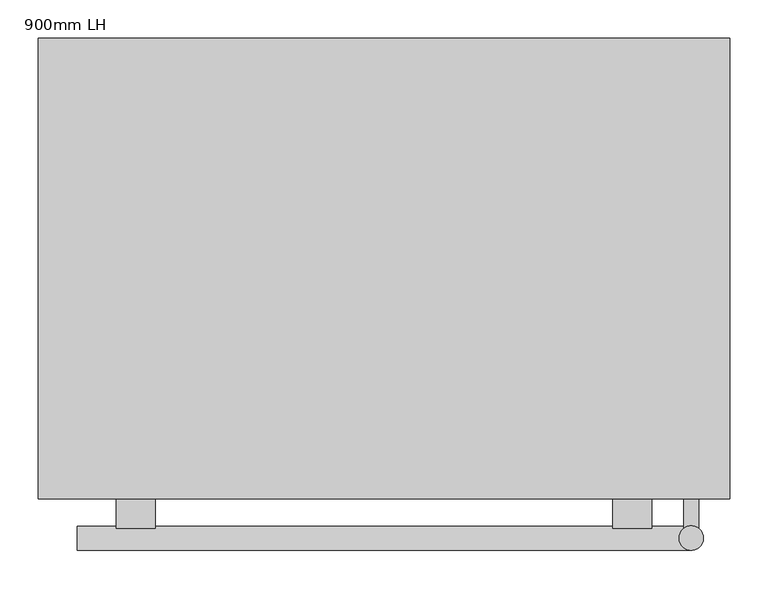
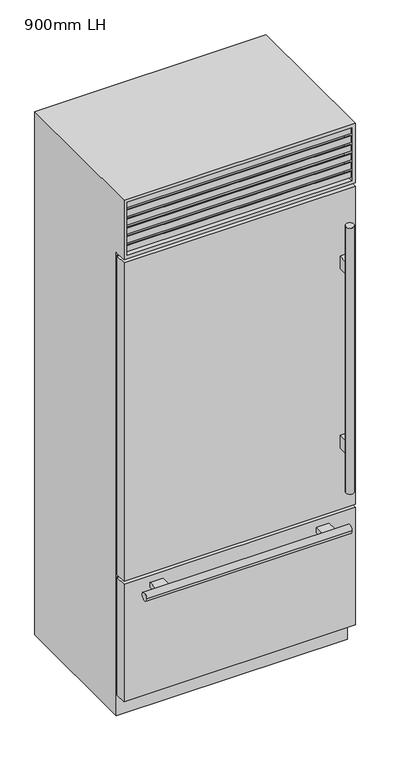
"""IFC4 building model written with IfcOpenShell, lengths in millimetres: proxy geometry, Refrigerador-combinado : 900mm LH."""

from ifc_helpers import new_model, si_unit, frame, origin, place, context, project, spatial, polyline, circle_curve, ellipse_curve, outline, extrude, faceted_brep, source, transform, mapped, element, save
from ifc_brep_helpers import plane_surface, cylinder_surface, advanced_brep


def proxy_900mm_lh_87200827(model_context):
    return source(origin(), model_context, "Body", "SolidModel", [
        extrude(outline(polyline([(-450.0, -655.55), (450.0, -655.55), (450.0, -700.0), (-450.0, -700.0), (-450.0, -655.55)])), frame((0.0, 0.0, 584.2), z_axis=(0.0, 0.0, 1.0), x_axis=(1.0, 0.0, 0.0)), (0.0, 0.0, 1.0), 1308.625),
        extrude(outline(polyline([(-450.0, -655.55), (450.0, -655.55), (450.0, -700.0), (-450.0, -700.0), (-450.0, -655.55)])), frame((0.0, 0.0, 88.9), z_axis=(0.0, 0.0, 1.0), x_axis=(1.0, 0.0, 0.0)), (0.0, 0.0, 1.0), 482.6),
        faceted_brep([(450.0, -700.0, 2150.0), (-450.0, -700.0, 2150.0), (-450.0, -700.0, 1905.525), (450.0, -700.0, 1905.525), (437.3, -700.0, 2137.3), (437.3, -700.0, 1918.225), (-437.3, -700.0, 1918.225), (-437.3, -700.0, 2137.3), (450.0, -100.0, 2150.0), (-450.0, -100.0, 2150.0), (-450.0, -100.0, 0.0), (-450.0, -649.2, 0.0), (-450.0, -649.2, 1905.525), (450.0, -649.2, 1905.525), (450.0, -649.2, 0.0), (450.0, -100.0, 0.0), (-437.3, -649.2, 2137.3), (437.3, -649.2, 2137.3), (-437.3, -649.2, 1918.225), (437.3, -649.2, 1918.225)], [[[0, 1, 2, 3], [4, 5, 6, 7]], [[1, 0, 8, 9]], [[2, 1, 9, 10, 11, 12]], [[3, 2, 12, 13]], [[8, 0, 3, 13, 14, 15]], [[4, 7, 16, 17]], [[7, 6, 18, 16]], [[6, 5, 19, 18]], [[5, 4, 17, 19]], [[15, 14, 11, 10]], [[9, 8, 15, 10]], [[17, 16, 18, 19]], [[11, 14, 13, 12]]]),
        extrude(outline(polyline([(-649.2, 1918.225), (-696.825, 1930.9860803), (-696.825, 1956.3860803), (-693.65, 1956.3860803), (-693.65, 1933.5368938), (-649.2, 1921.6265522), (-649.2, 1918.225)])), frame((-437.3, 0.0, 0.0), z_axis=(1.0, 0.0, 0.0), x_axis=(0.0, 1.0, 0.0)), (0.0, 0.0, 1.0), 874.6),
        extrude(outline(polyline([(-649.2, 1954.4077839), (-696.825, 1967.1688642), (-696.825, 1992.5688642), (-693.65, 1992.5688642), (-693.65, 1969.7196777), (-649.2, 1957.8093361), (-649.2, 1954.4077839)])), frame((-437.3, 0.0, 0.0), z_axis=(1.0, 0.0, 0.0), x_axis=(0.0, 1.0, 0.0)), (0.0, 0.0, 1.0), 874.6),
        extrude(outline(polyline([(-649.2, 1990.5905679), (-696.825, 2003.3516482), (-696.825, 2028.7516482), (-693.65, 2028.7516482), (-693.65, 2005.9024616), (-649.2, 1993.99212), (-649.2, 1990.5905679)])), frame((-437.3, 0.0, 0.0), z_axis=(1.0, 0.0, 0.0), x_axis=(0.0, 1.0, 0.0)), (0.0, 0.0, 1.0), 874.6),
        extrude(outline(polyline([(-649.2, 2026.7733518), (-696.825, 2039.5344321), (-696.825, 2064.9344321), (-693.65, 2064.9344321), (-693.65, 2042.0852456), (-649.2, 2030.174904), (-649.2, 2026.7733518)])), frame((-437.3, 0.0, 0.0), z_axis=(1.0, 0.0, 0.0), x_axis=(0.0, 1.0, 0.0)), (0.0, 0.0, 1.0), 874.6),
        extrude(outline(polyline([(-649.2, 2062.9561358), (-696.825, 2075.7172161), (-696.825, 2101.1172161), (-693.65, 2101.1172161), (-693.65, 2078.2680295), (-649.2, 2066.3576879), (-649.2, 2062.9561358)])), frame((-437.3, 0.0, 0.0), z_axis=(1.0, 0.0, 0.0), x_axis=(0.0, 1.0, 0.0)), (0.0, 0.0, 1.0), 874.6),
        extrude(outline(polyline([(-649.2, 2099.1389197), (-696.825, 2111.9), (-696.825, 2137.3), (-693.65, 2137.3), (-693.65, 2114.4508135), (-649.2, 2102.5404719), (-649.2, 2099.1389197)])), frame((-437.3, 0.0, 0.0), z_axis=(1.0, 0.0, 0.0), x_axis=(0.0, 1.0, 0.0)), (0.0, 0.0, 1.0), 874.6),
        advanced_brep(
        [(-443.65, -649.2, 565.15), (-443.65, -655.55, 565.15), (-443.65, -655.55, 95.25), (-443.65, -649.2, 95.25), (-446.825, -655.55, 568.325), (-446.825, -649.2, 568.325), (-446.825, -649.2, 92.075), (-446.825, -655.55, 92.075), (443.65, -655.55, 95.25), (443.65, -649.2, 95.25), (446.825, -649.2, 92.075), (446.825, -655.55, 92.075), (443.65, -655.55, 565.15), (443.65, -649.2, 565.15), (446.825, -649.2, 568.325), (446.825, -655.55, 568.325)],
        [
            (0, 1),
            (1, 2),
            (2, 3),
            (3, 0),
            (4, 5, ellipse_curve(frame((-446.825, -652.375, 568.325), z_axis=(-0.7071067811865475, 0.0, -0.7071067811865476), x_axis=(-0.7071067811865476, 0.0, 0.7071067811865475)), 4.4901281, 3.175)),
            (5, 6),
            (6, 7, ellipse_curve(frame((-446.825, -652.375, 92.075), z_axis=(-0.7071067811865475, 0.0, 0.7071067811865475), x_axis=(0.7071067811865474, 0.0, 0.7071067811865477)), 4.4901281, 3.175)),
            (7, 4),
            (2, 8),
            (8, 9),
            (9, 3),
            (6, 10),
            (10, 11, ellipse_curve(frame((446.825, -652.375, 92.075), z_axis=(-0.7071067811865475, 0.0, -0.7071067811865476), x_axis=(-0.7071067811865476, 0.0, 0.7071067811865474)), 4.4901281, 3.175)),
            (11, 7),
            (8, 12),
            (12, 13),
            (13, 9),
            (10, 14),
            (14, 15, ellipse_curve(frame((446.825, -652.375, 568.325), z_axis=(0.7071067811865476, 0.0, -0.7071067811865474), x_axis=(-0.7071067811865474, 0.0, -0.7071067811865477)), 4.4901281, 3.175)),
            (15, 11),
            (12, 1),
            (0, 13),
            (5, 14),
            (4, 15),
        ],
        [
            plane_surface(frame((-443.65, -655.55, 565.15), z_axis=(1.0, 0.0, 0.0), x_axis=(0.0, 0.0, -1.0))),
            cylinder_surface(frame((-446.825, -652.375, 571.5), z_axis=(0.0, 0.0, 1.0), x_axis=(0.0, -1.0, 0.0)), 3.175),
            plane_surface(frame((-443.65, -655.55, 95.25), z_axis=(0.0, 0.0, 1.0), x_axis=(1.0, 0.0, 0.0))),
            cylinder_surface(frame((-450.0, -652.375, 92.075), z_axis=(-1.0, 0.0, 0.0), x_axis=(0.0, -1.0, 0.0)), 3.175),
            plane_surface(frame((443.65, -655.55, 95.25), z_axis=(-1.0, 0.0, 0.0), x_axis=(0.0, 0.0, 1.0))),
            cylinder_surface(frame((446.825, -652.375, 88.9), z_axis=(0.0, 0.0, -1.0), x_axis=(0.0, -1.0, 0.0)), 3.175),
            plane_surface(frame((443.65, -655.55, 565.15), z_axis=(0.0, 0.0, -1.0), x_axis=(-1.0, 0.0, 0.0))),
            plane_surface(frame((443.65, -649.2, 565.15), z_axis=(0.0, 1.0, 0.0), x_axis=(-1.0, 0.0, 0.0))),
            cylinder_surface(frame((450.0, -652.375, 568.325), z_axis=(1.0, 0.0, 0.0), x_axis=(0.0, -1.0, 0.0)), 3.175),
            plane_surface(frame((446.825, -655.55, 568.325), z_axis=(0.0, -1.0, 0.0), x_axis=(-1.0, 0.0, 0.0))),
        ],
        [
            (0, [[1, 2, 3, 4]]),
            (1, [[5, 6, 7, 8]]),
            (2, [[-3, 9, 10, 11]]),
            (3, [[-7, 12, 13, 14]]),
            (4, [[-10, 15, 16, 17]]),
            (5, [[-13, 18, 19, 20]]),
            (6, [[-16, 21, -1, 22]]),
            (7, [[23, -18, -12, -6], [-11, -17, -22, -4]]),
            (8, [[-19, -23, -5, 24]]),
            (9, [[-14, -20, -24, -8], [-21, -15, -9, -2]]),
        ],
    ),
        advanced_brep(
        [(-443.65, -649.2, 1886.475), (-443.65, -655.55, 1886.475), (-443.65, -655.55, 590.55), (-443.65, -649.2, 590.55), (-446.825, -655.55, 1889.65), (-446.825, -649.2, 1889.65), (-446.825, -649.2, 587.375), (-446.825, -655.55, 587.375), (443.65, -655.55, 590.55), (443.65, -649.2, 590.55), (446.825, -649.2, 587.375), (446.825, -655.55, 587.375), (443.65, -655.55, 1886.475), (443.65, -649.2, 1886.475), (446.825, -649.2, 1889.65), (446.825, -655.55, 1889.65)],
        [
            (0, 1),
            (1, 2),
            (2, 3),
            (3, 0),
            (4, 5, ellipse_curve(frame((-446.825, -652.375, 1889.65), z_axis=(-0.7071067811865476, 0.0, -0.7071067811865475), x_axis=(-0.7071067811865475, 0.0, 0.7071067811865475)), 4.4901281, 3.175)),
            (5, 6),
            (6, 7, ellipse_curve(frame((-446.825, -652.375, 587.375), z_axis=(-0.7071067811865475, 0.0, 0.7071067811865476), x_axis=(0.7071067811865475, 0.0, 0.7071067811865475)), 4.4901281, 3.175)),
            (7, 4),
            (2, 8),
            (8, 9),
            (9, 3),
            (6, 10),
            (10, 11, ellipse_curve(frame((446.825, -652.375, 587.375), z_axis=(-0.7071067811865476, 0.0, -0.7071067811865475), x_axis=(-0.7071067811865475, 0.0, 0.7071067811865475)), 4.4901281, 3.175)),
            (11, 7),
            (8, 12),
            (12, 13),
            (13, 9),
            (10, 14),
            (14, 15, ellipse_curve(frame((446.825, -652.375, 1889.65), z_axis=(0.7071067811865474, 0.0, -0.7071067811865476), x_axis=(-0.7071067811865475, 0.0, -0.7071067811865476)), 4.4901281, 3.175)),
            (15, 11),
            (12, 1),
            (0, 13),
            (5, 14),
            (4, 15),
        ],
        [
            plane_surface(frame((-443.65, -655.55, 1886.475), z_axis=(1.0, 0.0, 0.0), x_axis=(0.0, 0.0, -1.0))),
            cylinder_surface(frame((-446.825, -652.375, 1892.825), z_axis=(0.0, 0.0, 1.0), x_axis=(0.0, -1.0, 0.0)), 3.175),
            plane_surface(frame((-443.65, -655.55, 590.55), z_axis=(0.0, 0.0, 1.0), x_axis=(1.0, 0.0, 0.0))),
            cylinder_surface(frame((-450.0, -652.375, 587.375), z_axis=(-1.0, 0.0, 0.0), x_axis=(0.0, -1.0, 0.0)), 3.175),
            plane_surface(frame((443.65, -655.55, 590.55), z_axis=(-1.0, 0.0, 0.0), x_axis=(0.0, 0.0, 1.0))),
            cylinder_surface(frame((446.825, -652.375, 584.2), z_axis=(0.0, 0.0, -1.0), x_axis=(0.0, -1.0, 0.0)), 3.175),
            plane_surface(frame((443.65, -655.55, 1886.475), z_axis=(0.0, 0.0, -1.0), x_axis=(-1.0, 0.0, 0.0))),
            plane_surface(frame((443.65, -649.2, 1886.475), z_axis=(0.0, 1.0, 0.0), x_axis=(-1.0, 0.0, 0.0))),
            cylinder_surface(frame((450.0, -652.375, 1889.65), z_axis=(1.0, 0.0, 0.0), x_axis=(0.0, -1.0, 0.0)), 3.175),
            plane_surface(frame((446.825, -655.55, 1889.65), z_axis=(0.0, -1.0, 0.0), x_axis=(-1.0, 0.0, 0.0))),
        ],
        [
            (0, [[1, 2, 3, 4]]),
            (1, [[5, 6, 7, 8]]),
            (2, [[-3, 9, 10, 11]]),
            (3, [[-7, 12, 13, 14]]),
            (4, [[-10, 15, 16, 17]]),
            (5, [[-13, 18, 19, 20]]),
            (6, [[-16, 21, -1, 22]]),
            (7, [[23, -18, -12, -6], [-11, -17, -22, -4]]),
            (8, [[-19, -23, -5, 24]]),
            (9, [[-14, -20, -24, -8], [-21, -15, -9, -2]]),
        ],
    ),
        advanced_brep(
        [(-297.6, -700.0, 542.925), (-297.6, -700.0, 523.875), (-348.4, -700.0, 523.875), (-348.4, -700.0, 542.925), (297.6, -700.0, 542.925), (348.4, -700.0, 542.925), (348.4, -700.0, 523.875), (297.6, -700.0, 523.875), (-297.6, -738.4741958, 542.925), (-297.6, -735.2991958, 533.4), (-297.6, -738.4741958, 523.875), (-348.4, -738.4741958, 523.875), (-348.4, -735.2991958, 533.4), (-348.4, -738.4741958, 542.925), (297.6, -738.4741958, 542.925), (348.4, -738.4741958, 542.925), (348.4, -735.2991958, 533.4), (348.4, -738.4741958, 523.875), (297.6, -738.4741958, 523.875), (297.6, -735.2991958, 533.4), (399.2, -767.0491958, 533.4), (399.2, -735.2991958, 533.4), (-399.2, -767.0491958, 533.4), (-399.2, -735.2991958, 533.4)],
        [
            (0, 1),
            (1, 2),
            (2, 3),
            (3, 0),
            (4, 5),
            (5, 6),
            (6, 7),
            (7, 4),
            (0, 8),
            (8, 9, circle_curve(frame((-297.6, -751.1741958, 533.4), z_axis=(-1.0, 0.0, 0.0), x_axis=(0.0, 1.0, 0.0)), 15.875)),
            (9, 10, circle_curve(frame((-297.6, -751.1741958, 533.4), z_axis=(-1.0, 0.0, 0.0), x_axis=(0.0, 1.0, 0.0)), 15.875)),
            (10, 1),
            (10, 11),
            (11, 2),
            (11, 12, circle_curve(frame((-348.4, -751.1741958, 533.4), z_axis=(1.0, 0.0, 0.0), x_axis=(0.0, 1.0, 0.0)), 15.875)),
            (12, 13, circle_curve(frame((-348.4, -751.1741958, 533.4), z_axis=(1.0, 0.0, 0.0), x_axis=(0.0, 1.0, 0.0)), 15.875)),
            (13, 3),
            (13, 8),
            (4, 14),
            (14, 15),
            (15, 5),
            (15, 16, circle_curve(frame((348.4, -751.1741958, 533.4), z_axis=(-1.0, 0.0, 0.0), x_axis=(0.0, 1.0, 0.0)), 15.875)),
            (16, 17, circle_curve(frame((348.4, -751.1741958, 533.4), z_axis=(-1.0, 0.0, 0.0), x_axis=(0.0, 1.0, 0.0)), 15.875)),
            (17, 6),
            (17, 18),
            (18, 7),
            (18, 19, circle_curve(frame((297.6, -751.1741958, 533.4), z_axis=(1.0, 0.0, 0.0), x_axis=(0.0, 1.0, 0.0)), 15.875)),
            (19, 14, circle_curve(frame((297.6, -751.1741958, 533.4), z_axis=(1.0, 0.0, 0.0), x_axis=(0.0, 1.0, 0.0)), 15.875)),
            (20, 21, circle_curve(frame((399.2, -751.1741958, 533.4), z_axis=(1.0, 0.0, 0.0), x_axis=(0.0, 1.0, 0.0)), 15.875)),
            (21, 20, circle_curve(frame((399.2, -751.1741958, 533.4), z_axis=(1.0, 0.0, 0.0), x_axis=(0.0, 1.0, 0.0)), 15.875)),
            (22, 23, circle_curve(frame((-399.2, -751.1741958, 533.4), z_axis=(-1.0, 0.0, 0.0), x_axis=(0.0, 1.0, 0.0)), 15.875)),
            (23, 22, circle_curve(frame((-399.2, -751.1741958, 533.4), z_axis=(-1.0, 0.0, 0.0), x_axis=(0.0, 1.0, 0.0)), 15.875)),
            (20, 22),
            (23, 12),
            (9, 19),
            (16, 21),
        ],
        [
            plane_surface(frame((-297.6, -700.0, 542.925), z_axis=(0.0, 1.0, 0.0), x_axis=(0.0, 0.0, -1.0))),
            plane_surface(frame((-297.6, -700.0, 542.925), z_axis=(1.0, 0.0, 0.0), x_axis=(0.0, -1.0, 0.0))),
            plane_surface(frame((-297.6, -700.0, 523.875), z_axis=(0.0, 0.0, -1.0), x_axis=(0.0, -1.0, 0.0))),
            plane_surface(frame((-348.4, -700.0, 523.875), z_axis=(-1.0, 0.0, 0.0), x_axis=(0.0, -1.0, 0.0))),
            plane_surface(frame((-348.4, -700.0, 542.925), z_axis=(0.0, 0.0, 1.0), x_axis=(0.0, -1.0, 0.0))),
            plane_surface(frame((297.6, -700.0, 542.925), z_axis=(0.0, 0.0, 1.0), x_axis=(0.0, -1.0, 0.0))),
            plane_surface(frame((348.4, -700.0, 542.925), z_axis=(1.0, 0.0, 0.0), x_axis=(0.0, -1.0, 0.0))),
            plane_surface(frame((348.4, -700.0, 523.875), z_axis=(0.0, 0.0, -1.0), x_axis=(0.0, -1.0, 0.0))),
            plane_surface(frame((297.6, -700.0, 523.875), z_axis=(-1.0, 0.0, 0.0), x_axis=(0.0, -1.0, 0.0))),
            plane_surface(frame((399.2, -735.2991958, 533.4), z_axis=(1.0, 0.0, 0.0), x_axis=(0.0, 0.0, 1.0))),
            plane_surface(frame((-399.2, -735.2991958, 533.4), z_axis=(-1.0, 0.0, 0.0), x_axis=(0.0, 0.0, -1.0))),
            cylinder_surface(frame((-399.2, -751.1741958, 533.4), z_axis=(1.0, 0.0, 0.0), x_axis=(0.0, 1.0, 0.0)), 15.875),
        ],
        [
            (0, [[1, 2, 3, 4]]),
            (0, [[5, 6, 7, 8]]),
            (1, [[-1, 9, 10, 11, 12]]),
            (2, [[-2, -12, 13, 14]]),
            (3, [[-3, -14, 15, 16, 17]]),
            (4, [[-4, -17, 18, -9]]),
            (5, [[-5, 19, 20, 21]]),
            (6, [[-6, -21, 22, 23, 24]]),
            (7, [[-7, -24, 25, 26]]),
            (8, [[-8, -26, 27, 28, -19]]),
            (9, [[29, 30]]),
            (10, [[31, 32]]),
            (11, [[-29, 33, -32, 34, -15, -13, -11, 35, -27, -25, -23, 36]]),
            (11, [[-30, -36, -22, -20, -28, -35, -10, -18, -16, -34, -31, -33]]),
        ],
    ),
        advanced_brep(
        [(409.525, -700.0, 1626.125), (409.525, -700.0, 1575.325), (390.475, -700.0, 1575.325), (390.475, -700.0, 1626.125), (409.525, -700.0, 889.0), (409.525, -700.0, 838.2), (390.475, -700.0, 838.2), (390.475, -700.0, 889.0), (409.525, -738.4741958, 1626.125), (409.525, -738.4741958, 1575.325), (390.475, -738.4741958, 1575.325), (390.475, -738.4741958, 1626.125), (409.525, -738.4741958, 889.0), (409.525, -738.4741958, 838.2), (390.475, -738.4741958, 838.2), (390.475, -738.4741958, 889.0), (384.125, -751.1741958, 1778.525), (415.875, -751.1741958, 1778.525), (384.125, -751.1741958, 685.8), (415.875, -751.1741958, 685.8)],
        [
            (0, 1),
            (1, 2),
            (2, 3),
            (3, 0),
            (4, 5),
            (5, 6),
            (6, 7),
            (7, 4),
            (0, 8),
            (8, 9),
            (9, 1),
            (9, 10, circle_curve(frame((400.0, -751.1741958, 1575.325), z_axis=(0.0, 0.0, 1.0), x_axis=(1.0, 0.0, 0.0)), 15.875)),
            (10, 2),
            (10, 11),
            (11, 3),
            (11, 8, circle_curve(frame((400.0, -751.1741958, 1626.125), z_axis=(0.0, 0.0, -1.0), x_axis=(1.0, 0.0, 0.0)), 15.875)),
            (4, 12),
            (12, 13),
            (13, 5),
            (13, 14, circle_curve(frame((400.0, -751.1741958, 838.2), z_axis=(0.0, 0.0, 1.0), x_axis=(1.0, 0.0, 0.0)), 15.875)),
            (14, 6),
            (14, 15),
            (15, 7),
            (15, 12, circle_curve(frame((400.0, -751.1741958, 889.0), z_axis=(0.0, 0.0, -1.0), x_axis=(1.0, 0.0, 0.0)), 15.875)),
            (16, 17, circle_curve(frame((400.0, -751.1741958, 1778.525), z_axis=(0.0, 0.0, 1.0), x_axis=(1.0, 0.0, 0.0)), 15.875)),
            (17, 16, circle_curve(frame((400.0, -751.1741958, 1778.525), z_axis=(0.0, 0.0, 1.0), x_axis=(1.0, 0.0, 0.0)), 15.875)),
            (18, 19, circle_curve(frame((400.0, -751.1741958, 685.8), z_axis=(0.0, 0.0, -1.0), x_axis=(1.0, 0.0, 0.0)), 15.875)),
            (19, 18, circle_curve(frame((400.0, -751.1741958, 685.8), z_axis=(0.0, 0.0, -1.0), x_axis=(1.0, 0.0, 0.0)), 15.875)),
            (16, 18),
            (19, 17),
        ],
        [
            plane_surface(frame((409.525, -700.0, 1626.125), z_axis=(0.0, 1.0, 0.0), x_axis=(0.0, 0.0, -1.0))),
            plane_surface(frame((409.525, -700.0, 1626.125), z_axis=(1.0, 0.0, 0.0), x_axis=(0.0, -1.0, 0.0))),
            plane_surface(frame((409.525, -700.0, 1575.325), z_axis=(0.0, 0.0, -1.0), x_axis=(0.0, -1.0, 0.0))),
            plane_surface(frame((390.475, -700.0, 1575.325), z_axis=(-1.0, 0.0, 0.0), x_axis=(0.0, -1.0, 0.0))),
            plane_surface(frame((390.475, -700.0, 1626.125), z_axis=(0.0, 0.0, 1.0), x_axis=(0.0, -1.0, 0.0))),
            plane_surface(frame((409.525, -700.0, 889.0), z_axis=(1.0, 0.0, 0.0), x_axis=(0.0, -1.0, 0.0))),
            plane_surface(frame((409.525, -700.0, 838.2), z_axis=(0.0, 0.0, -1.0), x_axis=(0.0, -1.0, 0.0))),
            plane_surface(frame((390.475, -700.0, 838.2), z_axis=(-1.0, 0.0, 0.0), x_axis=(0.0, -1.0, 0.0))),
            plane_surface(frame((390.475, -700.0, 889.0), z_axis=(0.0, 0.0, 1.0), x_axis=(0.0, -1.0, 0.0))),
            plane_surface(frame((415.875, -751.1741958, 1778.525), z_axis=(0.0, 0.0, 1.0), x_axis=(0.0, 1.0, 0.0))),
            plane_surface(frame((415.875, -751.1741958, 685.8), z_axis=(0.0, 0.0, -1.0), x_axis=(0.0, -1.0, 0.0))),
            cylinder_surface(frame((400.0, -751.1741958, 685.8), z_axis=(0.0, 0.0, 1.0), x_axis=(1.0, 0.0, 0.0)), 15.875),
        ],
        [
            (0, [[1, 2, 3, 4]]),
            (0, [[5, 6, 7, 8]]),
            (1, [[-1, 9, 10, 11]]),
            (2, [[-2, -11, 12, 13]]),
            (3, [[-3, -13, 14, 15]]),
            (4, [[-4, -15, 16, -9]]),
            (5, [[-5, 17, 18, 19]]),
            (6, [[-6, -19, 20, 21]]),
            (7, [[-7, -21, 22, 23]]),
            (8, [[-8, -23, 24, -17]]),
            (9, [[25, 26]]),
            (10, [[27, 28]]),
            (11, [[-25, 29, -28, 30]]),
            (11, [[-26, -30, -27, -29], [-10, -16, -14, -12], [-18, -24, -22, -20]]),
        ],
    ),
    ])


if __name__ == "__main__":
    model = new_model("IFC4")
    model_context = context("Model", 3, world=origin())
    ifc_project = project(units=[si_unit("LENGTHUNIT", "METRE", prefix="MILLI")], contexts=[model_context])
    site = spatial("IfcSite", under=ifc_project)
    building = spatial("IfcBuilding", under=site)
    placement = place(None, origin())
    proxy_900mm_lh_shape = proxy_900mm_lh_87200827(model_context)
    element("IfcBuildingElementProxy", 1, Name="Refrigerador-combinado : 900mm LH", ObjectType="Refrigerador-combinado : 900mm LH", at=placement, inside=building, context=model_context, shape_type="MappedRepresentation", body=[
        mapped(proxy_900mm_lh_shape, transform((0.0, 0.0, 0.0), x_axis=(1.0, 0.0, 0.0), y_axis=(0.0, 1.0, 0.0), z_axis=(0.0, 0.0, 1.0))),
    ])
    save(model, "model.ifc")

# Revit data of these elements
# Type "Refrigerador-combinado : 900mm LH"
#   Legenda = "Refrigerador"
#   Description = "Refrigerador combinado"
#   Assembly Code = "E1090320"
#   Largura = 900 mm
#   Deslocamento de parede = 100 mm
#   Voltagem = 120 V
#   Consumo de energia = 1000 VA
#   Altura = 2150 mm
#   Linha de centro do puxador = 850 mm
#   Linear = 600 mm
#   Amperagem = 8.33333 A
#   Mostrar legenda = yes
#   RH = no
#   LH = yes
#   Junta = Eletrodoméstico – Junta
#   Acabamento do eletrodoméstico = Eletrodoméstico – Aço inoxidável
# Element 1 (IfcBuildingElementProxy, "Refrigerador-combinado : 900mm LH")
#   Materials on its faces: "Eletrodoméstico – Aço inoxidável", "Eletrodoméstico – Junta"
# Materials
#   "Eletrodoméstico – Junta": class "Diversos", colour RGB 234 234 234, transparency 0, Cost = 0
#   "Eletrodoméstico – Aço inoxidável": class "Metal", colour RGB 189 187 185, transparency 0, Description = "Aço inoxidável 18/8", Cost = 0
